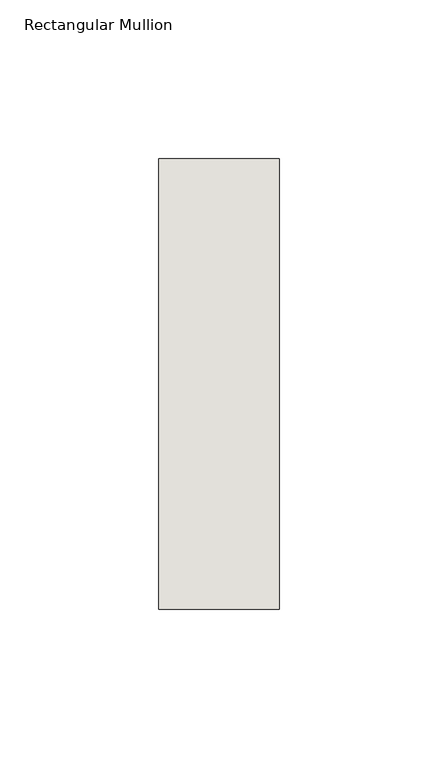
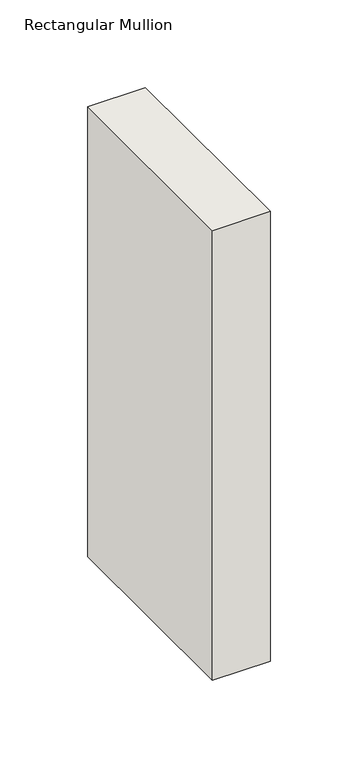
"""IFC4 building model written with IfcOpenShell, lengths in millimetres: wall geometry, Rectangular Mullion : NLRS_21_CWM_hsb-regel 38x142_gen_rsf."""

from ifc_helpers import new_model, si_unit, frame, origin, place, context, project, spatial, polyline, outline, extrude, source, transform, mapped, element, save


def rectangular_mullion_533ed1c3(model_context):
    return source(origin(), model_context, "Body", "SweptSolid", [
        extrude(outline(polyline([(-38.0, -71.0), (-38.0, 71.0), (0.0, 71.0), (0.0, -71.0), (-38.0, -71.0)])), frame((0.0, 0.0, -312.8441061), z_axis=(0.0, 0.0, 1.0), x_axis=(1.0, 0.0, 0.0)), (0.0, 0.0, 1.0), 312.8441061),
    ])


if __name__ == "__main__":
    model = new_model("IFC4")
    model_context = context("Model", 3, world=origin())
    ifc_project = project(units=[si_unit("LENGTHUNIT", "METRE", prefix="MILLI")], contexts=[model_context])
    site = spatial("IfcSite", under=ifc_project)
    building = spatial("IfcBuilding", under=site)
    placement = place(None, origin())
    rectangular_mullion_shape = rectangular_mullion_533ed1c3(model_context)
    element("IfcWall", 1, ObjectType="Rectangular Mullion : NLRS_21_CWM_hsb-regel 38x142_gen_rsf", at=placement, inside=building, context=model_context, shape_type="MappedRepresentation", body=[
        mapped(rectangular_mullion_shape, transform((0.0, 0.0, 0.0), x_axis=(1.0, 0.0, 0.0), y_axis=(0.0, 1.0, 0.0), z_axis=(0.0, 0.0, 1.0))),
    ])
    save(model, "model.ifc")

# Revit data of these elements
# Type "Rectangular Mullion : NLRS_21_CWM_hsb-regel 38x142_gen_rsf"
#   Type IfcGUID = "07M7mRoiH1CR8m_RSKIwpF"
#   Assembly Code = "21.10"
#   IfcExportAs = "IfcWall"
#   built-in parameter 1007322 = 0.465879 (stored number, unit not read)
#   built-in parameter 1007321 = 0.062336 (stored number, unit not read)
#   built-in parameter 1007320 = 0.062336 (stored number, unit not read)
# Element 1 (IfcWall, "Rectangular Mullion : NLRS_21_CWM_hsb-regel 38x142_gen_rsf")
#   Materials on its faces: "NLRS_i2_hout naaldhout vuren_gen_rsf"
# Materials
#   "NLRS_i2_hout naaldhout vuren_gen_rsf": class "I - Hout", colour RGB 234 199 147, transparency 0, Keynote = "i2", Manufacturer = "Revit Standards Foundation", URL = "www.revitstandards.org", Description = "hout vuren", Cost = 0
